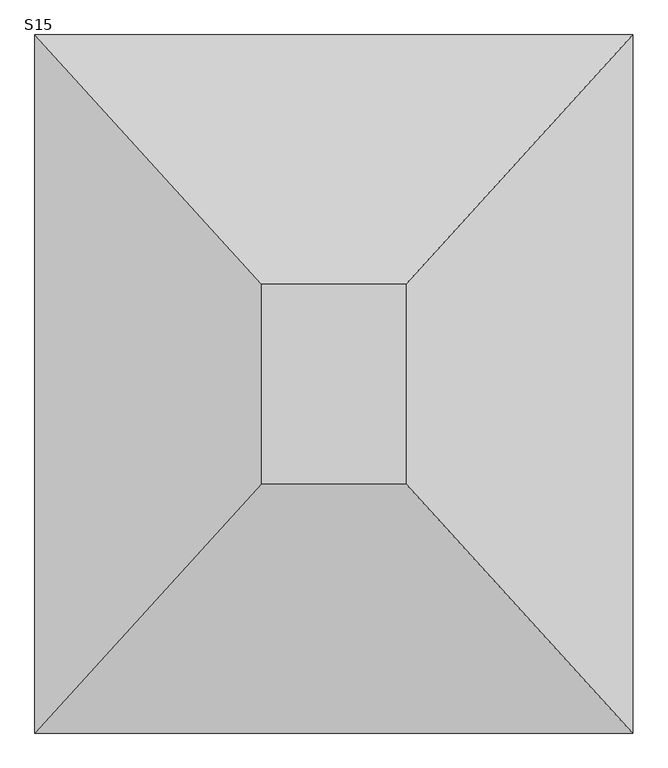
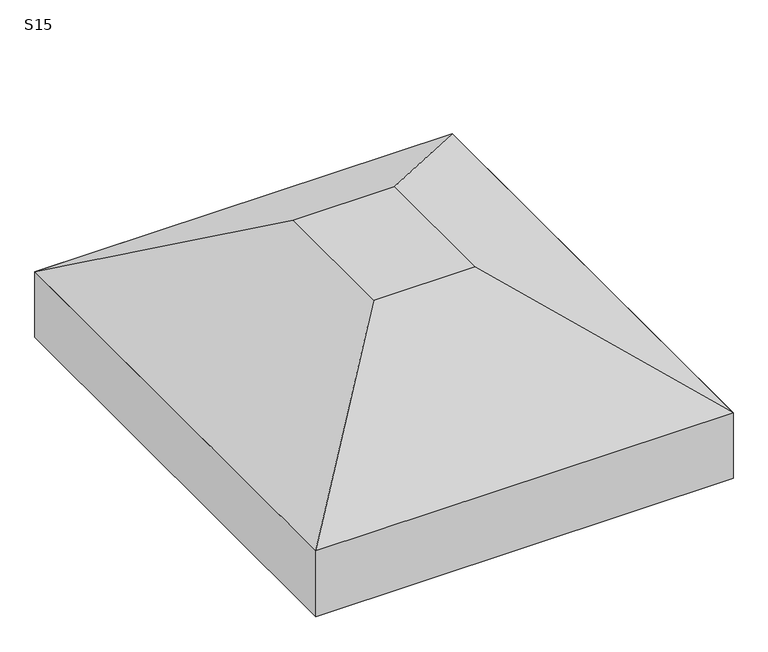
"""IFC4 building model written with IfcOpenShell, lengths in millimetres: fastener geometry, TQS - Sapata : S15."""

from ifc_helpers import new_model, si_unit, frame, origin, place, context, project, spatial, polyline, outline, extrude, faceted_brep, source, transform, mapped, element, save


def s15_bbe72304(model_context):
    return source(origin(), model_context, "Body", "SolidModel", [
        faceted_brep([(-55.0, 0.0, 0.0), (-345.0, 0.0, 0.0), (-345.0, -400.0, 0.0), (-55.0, -400.0, 0.0), (400.0, 500.0, -300.0), (400.0, -900.0, -300.0), (-800.0, -900.0, -300.0), (-800.0, 500.0, -300.0)], [[[0, 1, 2, 3]], [[4, 5, 6, 7]], [[4, 7, 1, 0]], [[7, 6, 2, 1]], [[6, 5, 3, 2]], [[5, 4, 0, 3]]]),
        extrude(outline(polyline([(400.0, 500.0), (400.0, -900.0), (-800.0, -900.0), (-800.0, 500.0), (400.0, 500.0)])), frame((0.0, 0.0, -500.0), z_axis=(0.0, 0.0, 1.0), x_axis=(1.0, 0.0, 0.0)), (0.0, 0.0, 1.0), 200.0),
    ])


if __name__ == "__main__":
    model = new_model("IFC4")
    model_context = context("Model", 3, world=origin())
    ifc_project = project(units=[si_unit("LENGTHUNIT", "METRE", prefix="MILLI")], contexts=[model_context])
    site = spatial("IfcSite", under=ifc_project)
    building = spatial("IfcBuilding", under=site)
    placement = place(None, origin())
    s15_shape = s15_bbe72304(model_context)
    element("IfcFastener", 1, ObjectType="TQS - Sapata : S15", at=placement, inside=building, context=model_context, shape_type="MappedRepresentation", body=[
        mapped(s15_shape, transform((0.0, 0.0, 0.0), x_axis=(1.0, 0.0, 0.0), y_axis=(0.0, 1.0, 0.0), z_axis=(0.0, 0.0, 1.0))),
    ])
    save(model, "model.ifc")

# Revit data of these elements
# Type "TQS - Sapata : S15"
#   TY = 0.40 m
#   TX = 0.29 m
#   HS = 0.50 m
#   H0 = 0.20 m
#   EXCYABS = 0.70 m
#   EXCY = 0.00 m
#   EXCXABS = 0.60 m
#   EXCX = 0.00 m
#   DIMY = 1.40 m
#   DIMX = 1.20 m
#   Material estrutural = Concreto - Concreto concretado no local
#   Width = 0
#   Length = 0
# Element 1 (IfcFastener, "TQS - Sapata : S15")
#   Materials on its faces: "Concreto - Concreto concretado no local"
# Materials
#   "Concreto - Concreto concretado no local": class "Concreto", colour RGB 192 192 192, transparency 0
